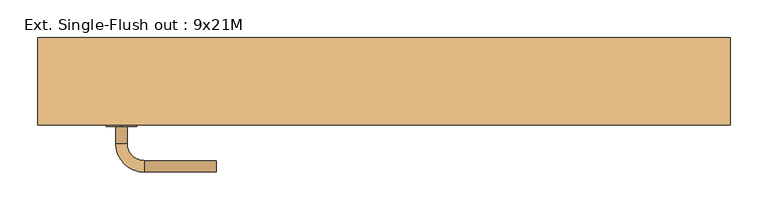
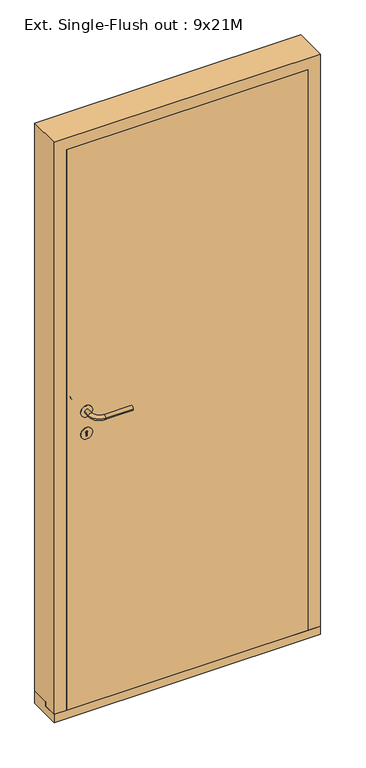
"""IFC4 building model written with IfcOpenShell, lengths in millimetres: door geometry, Ext. Single-Flush out : 9x21M."""

import ifcopenshell
import ifcopenshell.guid

model = None  # the IFC model being written
_history = None  # IfcOwnerHistory: only IFC2X3 demands one
_inside = {}  # id of a spatial element -> (the spatial element, [elements in it])
_under = {}  # id of a project, library or spatial element -> (it, [spatial elements below it])
_declared = {}  # id of a project -> (the project, [libraries it declares])
_typed = {}  # id of a type object -> (the type object, [elements of that type])
_made_of = {}  # id of a material, layer set ... -> (it, [elements and type objects made of it])


def new_model(schema):
    """Start an empty IFC model of exactly this schema.

    Asked for "IFC4X3", IfcOpenShell would pick the latest addendum, in which some entities
    have other attributes; the version numbers below select the first issue.
    IFC2X3 requires an IfcOwnerHistory on every rooted entity: one is made here for all.
    """
    global model, _history
    if schema == "IFC4X3":
        model = ifcopenshell.file(schema_version=(4, 3, 0, 0))
    else:
        model = ifcopenshell.file(schema=schema)
    _inside.clear()
    _under.clear()
    _declared.clear()
    _typed.clear()
    _made_of.clear()
    _history = None
    if model.schema == "IFC2X3":
        org = make("IfcOrganization", Name="unknown")
        user = make(
            "IfcPersonAndOrganization",
            ThePerson=make("IfcPerson", FamilyName="unknown"),
            TheOrganization=org,
        )
        app = make(
            "IfcApplication",
            ApplicationDeveloper=org,
            Version="unknown",
            ApplicationFullName="unknown",
            ApplicationIdentifier="unknown",
        )
        _history = make(
            "IfcOwnerHistory",
            OwningUser=user,
            OwningApplication=app,
            ChangeAction="ADDED",
            CreationDate=0,
        )
    return model


def make(cls, **values):
    """One entity of the class cls with the attributes given. An attribute that is None is left unset."""
    return model.create_entity(
        cls, **{name: value for name, value in values.items() if value is not None}
    )


def rooted(cls, **values):
    """An entity with a GlobalId (a new one), such as an element, a storey or a relation."""
    return make(cls, GlobalId=ifcopenshell.guid.new(), OwnerHistory=_history, **values)


def si_unit(unit_type, name, prefix=None):
    """IfcSIUnit, for example si_unit("LENGTHUNIT", "METRE", prefix="MILLI")."""
    return make("IfcSIUnit", UnitType=unit_type, Prefix=prefix, Name=name)


def assignment(units):
    """IfcUnitAssignment: the units of a project."""
    return None if units is None else make("IfcUnitAssignment", Units=units)


def point(xyz):
    """IfcCartesianPoint."""
    return None if xyz is None else make("IfcCartesianPoint", Coordinates=xyz)


def direction(xyz):
    """IfcDirection."""
    return None if xyz is None else make("IfcDirection", DirectionRatios=xyz)


def frame(location, z_axis=None, x_axis=None):
    """IfcAxis2Placement3D, a coordinate frame: its origin and axes. An axis left out is left unset."""
    return make(
        "IfcAxis2Placement3D",
        Location=point(location),
        Axis=direction(z_axis),
        RefDirection=direction(x_axis),
    )


def frame_2d(location, x_axis=None):
    """IfcAxis2Placement2D, a coordinate frame in the plane: its origin and x axis."""
    return make(
        "IfcAxis2Placement2D", Location=point(location), RefDirection=direction(x_axis)
    )


def origin():
    """The frame at (0, 0, 0) with its axes left unset."""
    return frame((0.0, 0.0, 0.0))


def place(relative_to, where):
    """IfcLocalPlacement: puts the frame where relative to a parent placement (None: the world)."""
    return make(
        "IfcLocalPlacement", PlacementRelTo=relative_to, RelativePlacement=where
    )


def context(
    kind, dimensions, precision=None, world=None, true_north=None, identifier=None
):
    """IfcGeometricRepresentationContext, for example the 3D "Model" context."""
    return make(
        "IfcGeometricRepresentationContext",
        ContextIdentifier=identifier,
        ContextType=kind,
        CoordinateSpaceDimension=dimensions,
        Precision=precision,
        WorldCoordinateSystem=world,
        TrueNorth=true_north,
    )


def project(units=None, contexts=None):
    """IfcProject with its units and contexts."""
    return rooted(
        "IfcProject",
        Name="project",
        RepresentationContexts=contexts,
        UnitsInContext=assignment(units),
    )


def spatial(cls, under=None, at=None, **own):
    """A site, building, storey or space (cls), placed at a placement, below another one or the project."""
    s = rooted(cls, ObjectPlacement=at, **own)
    if under is not None:
        _under.setdefault(under.id(), (under, []))[1].append(s)
    return s


def polyline(points):
    """IfcPolyline through the points."""
    return make("IfcPolyline", Points=[point(p) for p in points])


def circle_curve(where, radius):
    """IfcCircle in the frame where."""
    return make("IfcCircle", Position=where, Radius=radius)


def ellipse_curve(where, semi_axis1, semi_axis2):
    """IfcEllipse in the frame where."""
    return make(
        "IfcEllipse", Position=where, SemiAxis1=semi_axis1, SemiAxis2=semi_axis2
    )


def trimmed(basis, trim1, trim2, sense, master):
    """IfcTrimmedCurve: the piece of a basis curve between two trims."""
    return make(
        "IfcTrimmedCurve",
        BasisCurve=basis,
        Trim1=trim1,
        Trim2=trim2,
        SenseAgreement=sense,
        MasterRepresentation=master,
    )


def segment(curve, same_sense, transition):
    """IfcCompositeCurveSegment."""
    return make(
        "IfcCompositeCurveSegment",
        Transition=transition,
        SameSense=same_sense,
        ParentCurve=curve,
    )


def composite_curve(segments, self_intersect=None):
    """IfcCompositeCurve: segments joined end to end."""
    return make("IfcCompositeCurve", Segments=segments, SelfIntersect=self_intersect)


def outline(outer, holes=None, kind="AREA"):
    """IfcArbitraryClosedProfileDef: a profile drawn as a closed curve; with holes, ...WithVoids."""
    if holes is None:
        return make("IfcArbitraryClosedProfileDef", ProfileType=kind, OuterCurve=outer)
    return make(
        "IfcArbitraryProfileDefWithVoids",
        ProfileType=kind,
        OuterCurve=outer,
        InnerCurves=holes,
    )


def extrude(swept, where, along, depth):
    """IfcExtrudedAreaSolid: the profile swept, set in the frame where, extruded along a direction by depth."""
    return make(
        "IfcExtrudedAreaSolid",
        SweptArea=swept,
        Position=where,
        ExtrudedDirection=direction(along),
        Depth=depth,
    )


def faces_of(points, faces, orient=None, outer=None):
    """IfcFace entities. A face is a list of loops; a loop is a list of indices into points, from 0.

    orient and outer hold one flag for each loop. By default every Orientation is true, the
    first loop of a face is its IfcFaceOuterBound and the others are IfcFaceBound.
    """
    made = []
    for i, loops in enumerate(faces):
        bounds = []
        for j, loop in enumerate(loops):
            is_outer = j == 0 if outer is None else outer[i][j]
            bounds.append(
                make(
                    "IfcFaceOuterBound" if is_outer else "IfcFaceBound",
                    Bound=make("IfcPolyLoop", Polygon=[points[k] for k in loop]),
                    Orientation=True if orient is None else orient[i][j],
                )
            )
        made.append(make("IfcFace", Bounds=bounds))
    return made


def faceted_brep(points, faces, orient=None, outer=None, voids=None):
    """IfcFacetedBrep: a solid bounded by flat faces; with voids (closed shells), ...WithVoids."""
    shared = [point(p) for p in points]
    hull = make("IfcClosedShell", CfsFaces=faces_of(shared, faces, orient, outer))
    if voids is None:
        return make("IfcFacetedBrep", Outer=hull)
    return make(
        "IfcFacetedBrepWithVoids",
        Outer=hull,
        Voids=[
            make(cls, CfsFaces=faces_of(shared, fs, o, b)) for cls, fs, o, b in voids
        ],
    )


def shape(context_of_items, identifier, shape_type, items):
    """IfcShapeRepresentation: the items that make up one representation, for example the "Body"."""
    return make(
        "IfcShapeRepresentation",
        ContextOfItems=context_of_items,
        RepresentationIdentifier=identifier,
        RepresentationType=shape_type,
        Items=items,
    )


def source(mapping_origin, context_of_items, identifier, shape_type, items):
    """IfcRepresentationMap: a shape defined once, which mapped items show again and again."""
    return make(
        "IfcRepresentationMap",
        MappingOrigin=mapping_origin,
        MappedRepresentation=shape(context_of_items, identifier, shape_type, items),
    )


def transform(
    local_origin,
    x_axis=None,
    y_axis=None,
    z_axis=None,
    scale=None,
    scale2=None,
    scale3=None,
    uniform=True,
):
    """IfcCartesianTransformationOperator3D, or its non-uniform kind. x_axis, y_axis, z_axis: its Axis1, 2, 3."""
    if uniform:
        return make(
            "IfcCartesianTransformationOperator3D",
            Axis1=direction(x_axis),
            Axis2=direction(y_axis),
            LocalOrigin=point(local_origin),
            Scale=scale,
            Axis3=direction(z_axis),
        )
    return make(
        "IfcCartesianTransformationOperator3DnonUniform",
        Axis1=direction(x_axis),
        Axis2=direction(y_axis),
        LocalOrigin=point(local_origin),
        Scale=scale,
        Axis3=direction(z_axis),
        Scale2=scale2,
        Scale3=scale3,
    )


def mapped(mapping_source, mapping_target):
    """IfcMappedItem: shows the shape of a source again, moved by a transform."""
    return make(
        "IfcMappedItem", MappingSource=mapping_source, MappingTarget=mapping_target
    )


def made_of(thing, what):
    """Note that an element or type object is made of a material, layer set ...; save() writes the relation."""
    if what is not None:
        _made_of.setdefault(what.id(), (what, []))[1].append(thing)
    return thing


def element(
    cls,
    number,
    at=None,
    inside=None,
    cuts=None,
    type_object=None,
    material=None,
    context=None,
    identifier="Body",
    shape_type=None,
    held_by="IfcProductDefinitionShape",
    body=None,
    shapes=None,
    **own,
):
    """One element of the class cls, such as IfcWall. Its Tag is "e" and its number.

    at: its placement. inside: the storey or other place that contains it. cuts: it is an
    opening in that element (IfcRelVoidsElement). A single representation is given by context,
    identifier, shape_type and body (its items); several are given by shapes. held_by: the class
    of the entity that holds the representations. save() writes the other relations.
    """
    e = rooted(cls, Tag="e%d" % number, ObjectPlacement=at, **own)
    if body is not None:
        shapes = [shape(context, identifier, shape_type, body)]
    if shapes is not None:
        e.Representation = make(held_by, Representations=shapes)
    if inside is not None:
        _inside.setdefault(inside.id(), (inside, []))[1].append(e)
    if cuts is not None:
        rooted(
            "IfcRelVoidsElement", RelatingBuildingElement=cuts, RelatedOpeningElement=e
        )
    if type_object is not None:
        _typed.setdefault(type_object.id(), (type_object, []))[1].append(e)
    return made_of(e, material)


def aggregate(whole, parts):
    """IfcRelAggregates: a whole, such as a stair, and the parts it consists of."""
    return rooted("IfcRelAggregates", RelatingObject=whole, RelatedObjects=parts)


def save(model, path):
    """Write the relations noted so far, then the file.

    IfcRelAggregates (storeys below a building ...), IfcRelContainedInSpatialStructure (elements
    in a storey), IfcRelDefinesByType, IfcRelAssociatesMaterial and IfcRelDeclares: one each for
    every whole, place, type object, material and project.
    """
    for whole, parts in _under.values():
        aggregate(whole, parts)
    for where, things in _inside.values():
        rooted(
            "IfcRelContainedInSpatialStructure",
            RelatedElements=things,
            RelatingStructure=where,
        )
    for kind, things in _typed.values():
        rooted("IfcRelDefinesByType", RelatedObjects=things, RelatingType=kind)
    for what, things in _made_of.values():
        rooted("IfcRelAssociatesMaterial", RelatedObjects=things, RelatingMaterial=what)
    for by, libraries in _declared.values():
        rooted("IfcRelDeclares", RelatingContext=by, RelatedDefinitions=libraries)
    model.write(path)


def plane_surface(at):
    """IfcPlane: the flat surface through the origin of the frame at, square to its z axis."""
    return make("IfcPlane", Position=at)


def cylinder_surface(at, radius):
    """IfcCylindricalSurface: all points at the distance radius from the z axis of the frame at."""
    return make("IfcCylindricalSurface", Position=at, Radius=radius)


def revolved_surface(curve, axis_point, axis_direction):
    """IfcSurfaceOfRevolution: the curve turned about the line through axis_point along axis_direction."""
    return make(
        "IfcSurfaceOfRevolution",
        SweptCurve=make("IfcArbitraryOpenProfileDef", ProfileType="CURVE", Curve=curve),
        AxisPosition=make("IfcAxis1Placement", Location=point(axis_point), Axis=direction(axis_direction)),
    )


def advanced_brep(points, edges, surfaces, faces):
    """IfcAdvancedBrep: a solid bounded by faces that lie on surfaces and meet in shared edges.

    An edge is (start, end): straight between two places in points (the first is 0);
    or (start, end, curve); or (start, end, curve, False) where it runs against its curve.
    A face is (place in surfaces, loops), or (place, loops, False) where it looks against
    its surface's normal. A loop lists edges by number (the first is 1), with a minus sign
    where the edge is run from its end to its start. The first loop is the outer one.
    """
    corners = [point(p) for p in points]
    vertices = [make("IfcVertexPoint", VertexGeometry=c) for c in corners]
    made = []
    for start, end, *more in edges:
        made.append(
            make(
                "IfcEdgeCurve",
                EdgeStart=vertices[start],
                EdgeEnd=vertices[end],
                EdgeGeometry=more[0] if more else make("IfcPolyline", Points=[corners[start], corners[end]]),
                SameSense=more[1] if len(more) > 1 else True,
            )
        )
    hull = []
    for where, loops, *sense in faces:
        bounds = []
        for j, loop in enumerate(loops):
            ring = [make("IfcOrientedEdge", EdgeElement=made[abs(k) - 1], Orientation=k > 0) for k in loop]
            bounds.append(
                make(
                    "IfcFaceOuterBound" if j == 0 else "IfcFaceBound",
                    Bound=make("IfcEdgeLoop", EdgeList=ring),
                    Orientation=True,
                )
            )
        hull.append(make("IfcAdvancedFace", Bounds=bounds, FaceSurface=surfaces[where], SameSense=sense[0] if sense else True))
    return make("IfcAdvancedBrep", Outer=make("IfcClosedShell", CfsFaces=hull))


def ext_single_flush_out_9x21m_b425c0d5(model_context):
    return source(origin(), model_context, "Body", "SolidModel", [
        extrude(outline(composite_curve([segment(trimmed(circle_curve(frame_2d((1090.0, -346.0)), 20.0), [point((1070.0, -346.0))], [point((1110.0, -346.0))], False, "CARTESIAN"), True, "CONTINUOUS"), segment(trimmed(circle_curve(frame_2d((1090.0, -346.0)), 20.0), [point((1110.0, -346.0))], [point((1070.0, -346.0))], False, "CARTESIAN"), True, "CONTINUOUS")], self_intersect=False)), frame((0.0, -186.0, 0.0), z_axis=(0.0, 1.0, 0.0), x_axis=(0.0, 0.0, 1.0)), (0.0, 0.0, 1.0), 2.0),
        advanced_brep(
        [(-353.5, -186.0, 1090.0), (-338.5, -186.0, 1090.0), (-338.5, -208.5, 1090.0), (-353.5, -208.5, 1090.0), (-316.0, -231.0, 1090.0), (-316.0, -246.0, 1090.0), (-221.0, -231.0, 1090.0), (-221.0, -246.0, 1090.0)],
        [
            (0, 1, circle_curve(frame((-346.0, -186.0, 1090.0), z_axis=(0.0, 1.0, 0.0), x_axis=(1.0, 0.0, 0.0)), 7.5)),
            (1, 0, circle_curve(frame((-346.0, -186.0, 1090.0), z_axis=(0.0, 1.0, 0.0), x_axis=(1.0, 0.0, 0.0)), 7.5)),
            (1, 2),
            (2, 3, circle_curve(frame((-346.0, -208.5, 1090.0), z_axis=(0.0, 1.0, 0.0), x_axis=(1.0, 0.0, 0.0)), 7.5)),
            (3, 0),
            (3, 2, circle_curve(frame((-346.0, -208.5, 1090.0), z_axis=(0.0, 1.0, 0.0), x_axis=(1.0, 0.0, 0.0)), 7.5)),
            (4, 5, circle_curve(frame((-316.0, -238.5, 1090.0), z_axis=(-1.0, 0.0, 0.0), x_axis=(0.0, 1.0, 0.0)), 7.5)),
            (5, 3, circle_curve(frame((-316.0, -208.5, 1090.0), z_axis=(0.0, 0.0, -1.0), x_axis=(-1.0, 0.0, 0.0)), 37.5)),
            (2, 4, circle_curve(frame((-316.0, -208.5, 1090.0), z_axis=(0.0, 0.0, 1.0), x_axis=(-1.0, 0.0, 0.0)), 22.5)),
            (5, 4, circle_curve(frame((-316.0, -238.5, 1090.0), z_axis=(-1.0, 0.0, 0.0), x_axis=(0.0, 1.0, 0.0)), 7.5)),
            (4, 6),
            (6, 7, circle_curve(frame((-221.0, -238.5, 1090.0), z_axis=(-1.0, 0.0, 0.0), x_axis=(0.0, 1.0, 0.0)), 7.5)),
            (7, 5),
            (7, 6, circle_curve(frame((-221.0, -238.5, 1090.0), z_axis=(-1.0, 0.0, 0.0), x_axis=(0.0, 1.0, 0.0)), 7.5)),
        ],
        [
            plane_surface(frame((-346.0, -186.0, 1090.0), z_axis=(0.0, 1.0, 0.0), x_axis=(0.0, 0.0, -1.0))),
            cylinder_surface(frame((-346.0, -186.0, 1090.0), z_axis=(0.0, 1.0, 0.0), x_axis=(1.0, 0.0, 0.0)), 7.5),
            revolved_surface(trimmed(ellipse_curve(frame((-346.0, -208.5, 1090.0), z_axis=(0.0, -1.0, 0.0), x_axis=(1.0, 0.0, 0.0)), 7.5, 7.5), [point((-353.5, -208.5, 1090.0))], [point((-338.5, -208.5, 1090.0))], True, "CARTESIAN"), (-316.0, -208.5, 1090.0), (0.0, 0.0, -1.0)),
            revolved_surface(trimmed(ellipse_curve(frame((-346.0, -208.5, 1090.0), z_axis=(0.0, -1.0, 0.0), x_axis=(1.0, 0.0, 0.0)), 7.5, 7.5), [point((-338.5, -208.5, 1090.0))], [point((-353.5, -208.5, 1090.0))], True, "CARTESIAN"), (-316.0, -208.5, 1090.0), (0.0, 0.0, -1.0)),
            cylinder_surface(frame((-316.0, -238.5, 1090.0), z_axis=(-1.0, 0.0, 0.0), x_axis=(0.0, 1.0, 0.0)), 7.5),
            plane_surface(frame((-221.0, -238.5, 1090.0), z_axis=(1.0, 0.0, 0.0), x_axis=(0.0, 0.0, -1.0))),
        ],
        [
            (0, [[1, 2]]),
            (1, [[3, 4, 5, -2]]),
            (1, [[-5, 6, -3, -1]]),
            (2, [[7, 8, -4, 9]]),
            (3, [[10, -9, -6, -8]]),
            (4, [[11, 12, 13, -7]]),
            (4, [[-13, 14, -11, -10]]),
            (5, [[-12, -14]]),
        ],
    ),
        extrude(outline(composite_curve([segment(trimmed(circle_curve(frame_2d((1010.0, -346.0)), 20.0), [point((990.0, -346.0))], [point((1030.0, -346.0))], False, "CARTESIAN"), True, "CONTINUOUS"), segment(trimmed(circle_curve(frame_2d((1010.0, -346.0)), 20.0), [point((1030.0, -346.0))], [point((990.0, -346.0))], False, "CARTESIAN"), True, "CONTINUOUS")], self_intersect=False), holes=[composite_curve([segment(trimmed(circle_curve(frame_2d((1015.0, -346.0)), 3.0), [point((1012.4019238, -347.5))], [point((1012.4019238, -344.5))], True, "CARTESIAN"), True, "CONTINUOUS"), segment(polyline([(1012.4019238, -344.5), (1000.0, -344.5), (1000.0, -347.5), (1012.4019238, -347.5)]), True, "CONTINUOUS")], self_intersect=False)]), frame((0.0, -186.0, 0.0), z_axis=(0.0, 1.0, 0.0), x_axis=(0.0, 0.0, 1.0)), (0.0, 0.0, 1.0), 2.0),
        extrude(outline(composite_curve([segment(trimmed(circle_curve(frame_2d((1090.0, -346.0)), 20.0), [point((1070.0, -346.0))], [point((1110.0, -346.0))], False, "CARTESIAN"), True, "CONTINUOUS"), segment(trimmed(circle_curve(frame_2d((1090.0, -346.0)), 20.0), [point((1110.0, -346.0))], [point((1070.0, -346.0))], False, "CARTESIAN"), True, "CONTINUOUS")], self_intersect=False)), frame((0.0, -134.0, 0.0), z_axis=(0.0, 1.0, 0.0), x_axis=(0.0, 0.0, 1.0)), (0.0, 0.0, 1.0), 2.0),
        advanced_brep(
        [(-353.5, -132.0, 1090.0), (-338.5, -132.0, 1090.0), (-353.5, -109.5, 1090.0), (-338.5, -109.5, 1090.0), (-316.0, -87.0, 1090.0), (-316.0, -72.0, 1090.0), (-221.0, -72.0, 1090.0), (-221.0, -87.0, 1090.0)],
        [
            (0, 1, circle_curve(frame((-346.0, -132.0, 1090.0), z_axis=(0.0, -1.0, 0.0), x_axis=(1.0, 0.0, 0.0)), 7.5)),
            (1, 0, circle_curve(frame((-346.0, -132.0, 1090.0), z_axis=(0.0, -1.0, 0.0), x_axis=(1.0, 0.0, 0.0)), 7.5)),
            (0, 2),
            (2, 3, circle_curve(frame((-346.0, -109.5, 1090.0), z_axis=(0.0, -1.0, 0.0), x_axis=(1.0, 0.0, 0.0)), 7.5)),
            (3, 1),
            (3, 2, circle_curve(frame((-346.0, -109.5, 1090.0), z_axis=(0.0, -1.0, 0.0), x_axis=(1.0, 0.0, 0.0)), 7.5)),
            (4, 3, circle_curve(frame((-316.0, -109.5, 1090.0), z_axis=(0.0, 0.0, 1.0), x_axis=(-1.0, 0.0, 0.0)), 22.5)),
            (2, 5, circle_curve(frame((-316.0, -109.5, 1090.0), z_axis=(0.0, 0.0, -1.0), x_axis=(-1.0, 0.0, 0.0)), 37.5)),
            (5, 4, circle_curve(frame((-316.0, -79.5, 1090.0), z_axis=(-1.0, 0.0, 0.0), x_axis=(0.0, -1.0, 0.0)), 7.5)),
            (4, 5, circle_curve(frame((-316.0, -79.5, 1090.0), z_axis=(-1.0, 0.0, 0.0), x_axis=(0.0, -1.0, 0.0)), 7.5)),
            (5, 6),
            (6, 7, circle_curve(frame((-221.0, -79.5, 1090.0), z_axis=(-1.0, 0.0, 0.0), x_axis=(0.0, -1.0, 0.0)), 7.5)),
            (7, 4),
            (7, 6, circle_curve(frame((-221.0, -79.5, 1090.0), z_axis=(-1.0, 0.0, 0.0), x_axis=(0.0, -1.0, 0.0)), 7.5)),
        ],
        [
            plane_surface(frame((-346.0, -132.0, 1090.0), z_axis=(0.0, -1.0, 0.0), x_axis=(0.0, 0.0, -1.0))),
            cylinder_surface(frame((-346.0, -132.0, 1090.0), z_axis=(0.0, -1.0, 0.0), x_axis=(1.0, 0.0, 0.0)), 7.5),
            revolved_surface(trimmed(ellipse_curve(frame((-346.0, -109.5, 1090.0), z_axis=(0.0, -1.0, 0.0), x_axis=(1.0, 0.0, 0.0)), 7.5, 7.5), [point((-353.5, -109.5, 1090.0))], [point((-338.5, -109.5, 1090.0))], True, "CARTESIAN"), (-316.0, -109.5, 1090.0), (0.0, 0.0, -1.0)),
            revolved_surface(trimmed(ellipse_curve(frame((-346.0, -109.5, 1090.0), z_axis=(0.0, -1.0, 0.0), x_axis=(1.0, 0.0, 0.0)), 7.5, 7.5), [point((-338.5, -109.5, 1090.0))], [point((-353.5, -109.5, 1090.0))], True, "CARTESIAN"), (-316.0, -109.5, 1090.0), (0.0, 0.0, -1.0)),
            cylinder_surface(frame((-316.0, -79.5, 1090.0), z_axis=(-1.0, 0.0, 0.0), x_axis=(0.0, -1.0, 0.0)), 7.5),
            plane_surface(frame((-221.0, -79.5, 1090.0), z_axis=(1.0, 0.0, 0.0), x_axis=(0.0, 0.0, -1.0))),
        ],
        [
            (0, [[1, 2]]),
            (1, [[-1, 3, 4, 5]]),
            (1, [[-2, -5, 6, -3]]),
            (2, [[7, -4, 8, 9]]),
            (3, [[-8, -6, -7, 10]]),
            (4, [[-9, 11, 12, 13]]),
            (4, [[-10, -13, 14, -11]]),
            (5, [[-14, -12]]),
        ],
    ),
        extrude(outline(composite_curve([segment(trimmed(circle_curve(frame_2d((1010.0, -346.0)), 20.0), [point((990.0, -346.0))], [point((1030.0, -346.0))], False, "CARTESIAN"), True, "CONTINUOUS"), segment(trimmed(circle_curve(frame_2d((1010.0, -346.0)), 20.0), [point((1030.0, -346.0))], [point((990.0, -346.0))], False, "CARTESIAN"), True, "CONTINUOUS")], self_intersect=False), holes=[composite_curve([segment(trimmed(circle_curve(frame_2d((1015.0, -346.0)), 3.0), [point((1012.4019238, -347.5))], [point((1012.4019238, -344.5))], True, "CARTESIAN"), True, "CONTINUOUS"), segment(polyline([(1012.4019238, -344.5), (1000.0, -344.5), (1000.0, -347.5), (1012.4019238, -347.5)]), True, "CONTINUOUS")], self_intersect=False)]), frame((0.0, -134.0, 0.0), z_axis=(0.0, 1.0, 0.0), x_axis=(0.0, 0.0, 1.0)), (0.0, 0.0, 1.0), 2.0),
        extrude(outline(polyline([(-414.0, -184.0), (-414.0, -134.0), (414.0, -134.0), (414.0, -184.0), (-414.0, -184.0)])), frame((0.0, 0.0, 30.0), z_axis=(0.0, 0.0, 1.0), x_axis=(1.0, 0.0, 0.0)), (0.0, 0.0, 1.0), 2028.0),
        faceted_brep([(414.0, -184.0, 2058.0), (414.0, -184.0, 30.0), (456.0, -184.0, 30.0), (456.0, -184.0, 2100.0), (-456.0, -184.0, 2100.0), (-456.0, -184.0, 30.0), (-414.0, -184.0, 30.0), (-414.0, -184.0, 2058.0), (-414.0, -134.0, 30.0), (-414.0, -134.0, 45.0), (-414.0, -134.0, 2058.0), (-456.0, -134.0, 30.0), (456.0, -134.0, 30.0), (414.0, -134.0, 30.0), (-456.0, -69.0, 2100.0), (-456.0, -69.0, 45.0), (-456.0, -134.0, 45.0), (456.0, -134.0, 45.0), (456.0, -69.0, 45.0), (456.0, -69.0, 2100.0), (414.0, -134.0, 2058.0), (414.0, -134.0, 45.0), (399.0, -69.0, 45.0), (399.0, -69.0, 2043.0), (-399.0, -69.0, 2043.0), (-399.0, -69.0, 45.0), (-399.0, -134.0, 45.0), (399.0, -134.0, 45.0), (-399.0, -134.0, 2043.0), (399.0, -134.0, 2043.0)], [[[0, 1, 2, 3, 4, 5, 6, 7]], [[7, 6, 8, 9, 10]], [[8, 6, 5, 11]], [[12, 2, 1, 13]], [[14, 15, 16, 11, 5, 4]], [[3, 2, 12, 17, 18, 19]], [[20, 21, 13, 1, 0]], [[19, 18, 22, 23, 24, 25, 15, 14]], [[16, 15, 25, 26, 9]], [[21, 27, 22, 18, 17]], [[9, 8, 11, 16]], [[17, 12, 13, 21]], [[28, 26, 25, 24]], [[23, 22, 27, 29]], [[29, 27, 21, 20, 10, 9, 26, 28]], [[3, 19, 14, 4]], [[23, 29, 28, 24]], [[7, 10, 20, 0]]]),
        extrude(outline(polyline([(-184.0, 30.0), (-134.0, 30.0), (-134.0, 45.0), (-69.0, 45.0), (-69.0, 0.0), (-184.0, 0.0), (-184.0, 30.0)])), frame((-456.0, 0.0, 0.0), z_axis=(1.0, 0.0, 0.0), x_axis=(0.0, 1.0, 0.0)), (0.0, 0.0, 1.0), 912.0),
    ])


if __name__ == "__main__":
    model = new_model("IFC4")
    model_context = context("Model", 3, world=origin())
    ifc_project = project(units=[si_unit("LENGTHUNIT", "METRE", prefix="MILLI")], contexts=[model_context])
    site = spatial("IfcSite", under=ifc_project)
    building = spatial("IfcBuilding", under=site)
    placement = place(None, origin())
    ext_single_flush_out_9x21m_shape = ext_single_flush_out_9x21m_b425c0d5(model_context)
    element("IfcDoor", 1, ObjectType="Ext. Single-Flush out : 9x21M", at=placement, inside=building, context=model_context, shape_type="MappedRepresentation", body=[
        mapped(ext_single_flush_out_9x21m_shape, transform((0.0, 0.0, 0.0), x_axis=(1.0, 0.0, 0.0), y_axis=(0.0, 1.0, 0.0), z_axis=(0.0, 0.0, 1.0))),
    ])
    save(model, "model.ifc")

# Revit data of these elements
# Type "Ext. Single-Flush out : 9x21M"
#   Type Mark = "63"
#   Sound Rating = ""
#   Opening Side [instance default] = "out"
#   Hinge Side [instance default] = ""
#   Creator Organization [instance default] = "© Danish Educational Content"
#   Creator Name [instance default] = "© Erik Falck Jørgensen"
#   Creator Build [instance default] = "2017.0301.0"
#   Analytic Construction = "<None>"
#   length#6 = -50 mm
#   length#4 = 120 mm
#   length#5 = 912 mm
#   length#3 = 30 mm
#   length#2 = 57 mm
#   length#1 = 0 mm
#   Thickness = 50 mm
#   Seal Width = 12 mm
#   Rough Width = 912 mm
#   Rough Height = 2100 mm
#   Rebate Depth = 50 mm
#   Rabbet Width = 15 mm
#   Rabbet Depth = 50 mm
#   Height = 2088 mm
#   Width = 888 mm
#   Handle From Side = 110 mm
#   Handle From Bottom = 1090 mm
#   Exterior Direction [instance default] = 0.00°
#   Case Depth = 115 mm
#   Case Width = 45 mm
#   Threshold = yes
#   Sealing = no
#   Hinging = yes
#   Wall Closure = 1
#   Function = 1
#   Panel = none
#   Handle Finish = none
#   Handle = element 632149
#   Case/Transom = none
#   Assembly Code = ""
# Element 1 (IfcDoor, "Ext. Single-Flush out : 9x21M")
#   Materials on its faces: "Stainless Steel, Polished", "Default Frame/Mullion (Interior/Exterior)", "Default Door Panel (Exterior/Interior)"
# Materials
#   "Stainless Steel, Polished": class "Metal", colour RGB 180 180 180, transparency 0, Description = "Rustfri stål, poleret", Cost = 0
#   "Default Frame/Mullion (Interior/Exterior)": class "Generic", colour RGB 205 205 205, transparency 0, Description = "Udefineret karm/ramme materiale", Cost = 0
#   "Default Door Panel (Exterior/Interior)": class "Generic", colour RGB 205 205 205, transparency 0, Description = "Udefineret dørplade materiale", Cost = 0
